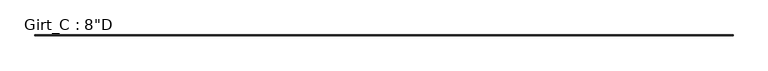
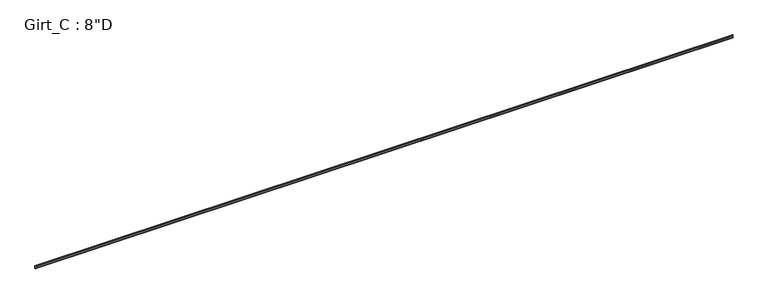
"""IFC4 building model written with IfcOpenShell, lengths in millimetres: beam geometry."""

from ifc_helpers import new_model, si_unit, point, frame, frame_2d, origin, place, context, project, spatial, polyline, circle_curve, trimmed, segment, composite_curve, outline, extrude, source, transform, mapped, element, save


def beam_ef5cc90a(model_context):
    return source(origin(), model_context, "Body", "SweptSolid", [
        extrude(outline(composite_curve([segment(polyline([(-63.5, 101.6), (-3.3734375, 101.6)]), True, "CONTINUOUS"), segment(trimmed(circle_curve(frame_2d((-3.3734375, 96.8375)), 4.7625), [point((-3.3734375, 101.6))], [point((1.3890625, 96.8375))], False, "CARTESIAN"), True, "CONTINUOUS"), segment(polyline([(1.3890625, 96.8375), (1.3890625, -96.8375)]), True, "CONTINUOUS"), segment(trimmed(circle_curve(frame_2d((-3.3734375, -96.8375)), 4.7625), [point((1.3890625, -96.8375))], [point((-3.3734375, -101.6))], False, "CARTESIAN"), True, "CONTINUOUS"), segment(polyline([(-3.3734375, -101.6), (-63.5, -101.6), (-75.745104, -87.0068534), (-73.6169367, -85.221109), (-62.204539, -98.821875), (-3.2694106, -98.821875)]), True, "CONTINUOUS"), segment(trimmed(circle_curve(frame_2d((-3.3748024, -96.8389339)), 1.9857399), [point((-3.2694106, -98.821875))], [point((-1.3890625, -96.8389339))], True, "CARTESIAN"), True, "CONTINUOUS"), segment(polyline([(-1.3890625, -96.8389339), (-1.3890625, 96.8381931)]), True, "CONTINUOUS"), segment(trimmed(circle_curve(frame_2d((-3.3741066, 96.8381931)), 1.9850441), [point((-1.3890625, 96.8381931))], [point((-3.3005807, 98.821875))], True, "CARTESIAN"), True, "CONTINUOUS"), segment(polyline([(-3.3005807, 98.821875), (-62.204539, 98.821875), (-73.6169367, 85.221109), (-75.745104, 87.0068534), (-63.5, 101.6)]), True, "CONTINUOUS")], self_intersect=False)), frame((-26733.5, 0.0, 0.0), z_axis=(1.0, 0.0, 0.0), x_axis=(0.0, 1.0, 0.0)), (0.0, 0.0, 1.0), 53467.0),
    ])


if __name__ == "__main__":
    model = new_model("IFC4")
    model_context = context("Model", 3, world=origin())
    ifc_project = project(units=[si_unit("LENGTHUNIT", "METRE", prefix="MILLI")], contexts=[model_context])
    site = spatial("IfcSite", under=ifc_project)
    building = spatial("IfcBuilding", under=site)
    placement = place(None, origin())
    beam_shape = beam_ef5cc90a(model_context)
    element("IfcBeam", 1, ObjectType="Girt_C : 8\"D", at=placement, inside=building, context=model_context, shape_type="MappedRepresentation", body=[
        mapped(beam_shape, transform((0.0, 0.0, 0.0), x_axis=(1.0, 0.0, 0.0), y_axis=(0.0, 1.0, 0.0), z_axis=(0.0, 0.0, 1.0))),
    ])
    save(model, "model.ifc")

# Revit data of these elements
# Type "Girt_C : 8\"D"
#   Web_Thickness = 0' - 0 7/64"
#   Length [instance default] = 10' - 0"
#   Leg_1 = 0' - 2 1/2"
#   Height = 0' - 8"
#   Structural Material [instance default] = none
# Element 1 (IfcBeam, "Girt_C : 8\"D")
#   Structural Material = Steel
#   Materials on its faces: "Steel"
# Materials
#   "Steel": class "Metal", colour RGB 118 118 114, transparency 0, Description = "Steel, mill finish", Cost = 0
